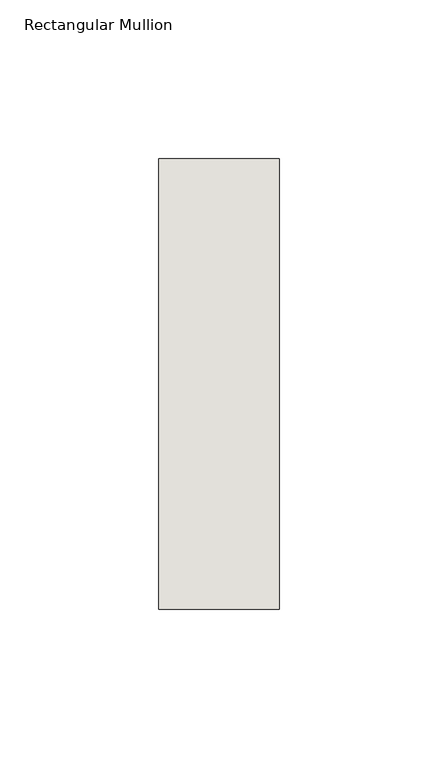
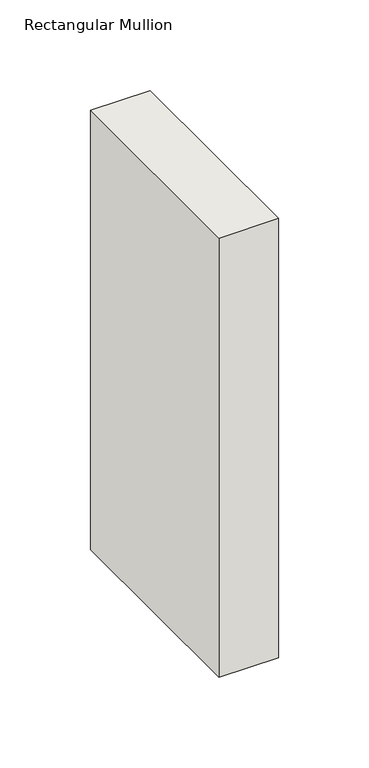
"""IFC4 building model written with IfcOpenShell, lengths in millimetres: wall geometry, Rectangular Mullion : NLRS_21_CWM_hsb-regel 38x142_gen_rsf."""

from ifc_helpers import new_model, si_unit, frame, origin, place, context, project, spatial, polyline, outline, extrude, source, transform, mapped, element, save


def rectangular_mullion_567310a4(model_context):
    return source(origin(), model_context, "Body", "SweptSolid", [
        extrude(outline(polyline([(0.0, -71.0), (-38.0, -71.0), (-38.0, 71.0), (0.0, 71.0), (0.0, -71.0)])), frame((0.0, 0.0, -296.0), z_axis=(0.0, 0.0, 1.0), x_axis=(1.0, 0.0, 0.0)), (0.0, 0.0, 1.0), 296.0),
    ])


if __name__ == "__main__":
    model = new_model("IFC4")
    model_context = context("Model", 3, world=origin())
    ifc_project = project(units=[si_unit("LENGTHUNIT", "METRE", prefix="MILLI")], contexts=[model_context])
    site = spatial("IfcSite", under=ifc_project)
    building = spatial("IfcBuilding", under=site)
    placement = place(None, origin())
    rectangular_mullion_shape = rectangular_mullion_567310a4(model_context)
    element("IfcWall", 1, ObjectType="Rectangular Mullion : NLRS_21_CWM_hsb-regel 38x142_gen_rsf", at=placement, inside=building, context=model_context, shape_type="MappedRepresentation", body=[
        mapped(rectangular_mullion_shape, transform((0.0, 0.0, 0.0), x_axis=(1.0, 0.0, 0.0), y_axis=(0.0, 1.0, 0.0), z_axis=(0.0, 0.0, 1.0))),
    ])
    save(model, "model.ifc")

# Revit data of these elements
# Type "Rectangular Mullion : NLRS_21_CWM_hsb-regel 38x142_gen_rsf"
#   Type IfcGUID = "07M7mRoiH1CR8m_RSKIwpF"
#   Assembly Code = "21.10"
#   IfcExportAs = "IfcWall"
#   built-in parameter 1007322 = 0.465879 (stored number, unit not read)
#   built-in parameter 1007321 = 0.062336 (stored number, unit not read)
#   built-in parameter 1007320 = 0.062336 (stored number, unit not read)
# Element 1 (IfcWall, "Rectangular Mullion : NLRS_21_CWM_hsb-regel 38x142_gen_rsf")
#   Materials on its faces: "NLRS_i2_hout naaldhout vuren_gen_rsf"
# Materials
#   "NLRS_i2_hout naaldhout vuren_gen_rsf": class "I - Hout", colour RGB 234 199 147, transparency 0, Keynote = "i2", Manufacturer = "Revit Standards Foundation", URL = "www.revitstandards.org", Description = "hout vuren", Cost = 0
